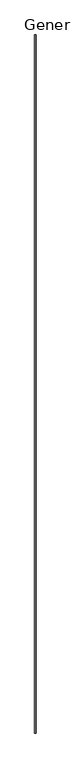
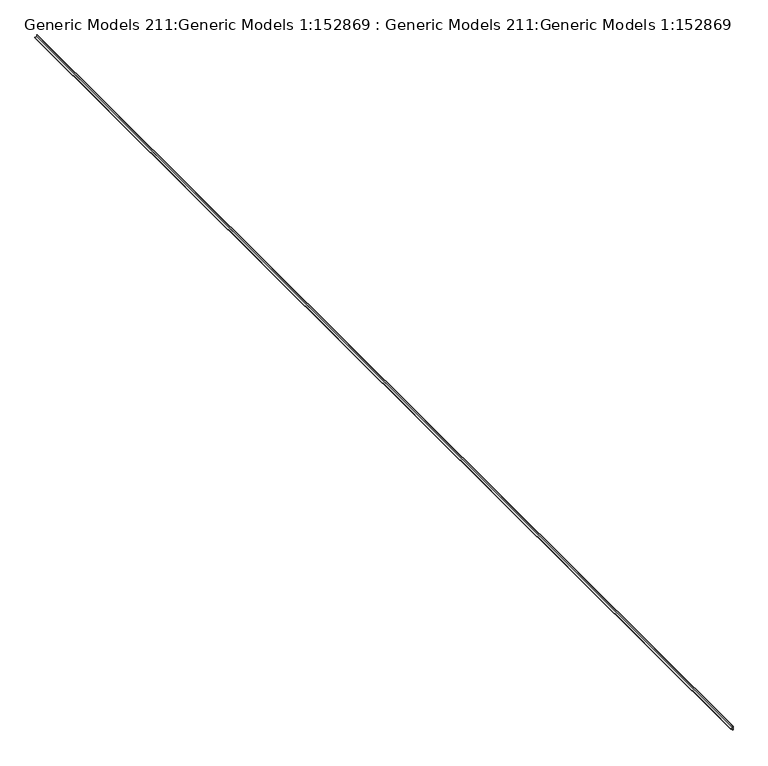
"""IFC4 building model written with IfcOpenShell, lengths in millimetres: proxy geometry, Generic Models 211:Generic Models 1:152869 : Generic Models 211:Generic Models 1:152869."""

from ifc_helpers import new_model, si_unit, frame, origin, place, context, project, spatial, polyline, outline, extrude, source, transform, mapped, element, save


def generic_models_211_generic_models_1_152869_generic_models_dbfa076a(model_context):
    return source(origin(), model_context, "Body", "SweptSolid", [
        extrude(outline(polyline([(3005.455, -6667.0793913), (3044.825, -6667.0793913), (3044.825, -6668.3493913), (3025.775, -6668.3493913), (3025.775, -6689.3043913), (3021.0252, -6689.3043913), (3021.0252, -6688.0343913), (3024.505, -6688.0343913), (3024.505, -6668.3493913), (3005.455, -6668.3493913), (3005.455, -6667.0793913)])), frame((0.0, -273.9974793, 0.0), z_axis=(0.0, 1.0, 0.0), x_axis=(0.0, 0.0, 1.0)), (0.0, 0.0, 1.0), 12446.0),
    ])


if __name__ == "__main__":
    model = new_model("IFC4")
    model_context = context("Model", 3, world=origin())
    ifc_project = project(units=[si_unit("LENGTHUNIT", "METRE", prefix="MILLI")], contexts=[model_context])
    site = spatial("IfcSite", under=ifc_project)
    building = spatial("IfcBuilding", under=site)
    placement = place(None, origin())
    generic_models_211_generic_models_1_152869_generic_models_shape = generic_models_211_generic_models_1_152869_generic_models_dbfa076a(model_context)
    element("IfcBuildingElementProxy", 1, Name="Generic Models 211:Generic Models 1:152869 : Generic Models 211:Generic Models 1:152869", ObjectType="Generic Models 211:Generic Models 1:152869 : Generic Models 211:Generic Models 1:152869", at=placement, inside=building, context=model_context, shape_type="MappedRepresentation", body=[
        mapped(generic_models_211_generic_models_1_152869_generic_models_shape, transform((0.0, 0.0, 0.0), x_axis=(1.0, 0.0, 0.0), y_axis=(0.0, 1.0, 0.0), z_axis=(0.0, 0.0, 1.0))),
    ])
    save(model, "model.ifc")

# Revit data of these elements
# Type "Generic Models 211:Generic Models 1:152869 : Generic Models 211:Generic Models 1:152869"
#   NameOverride = "Generic Models 211:Generic Models 1:152869"
#   ObjectTypeOverride = "Generic Models 211:Generic Models 1"
#   Reference = "Generic Models 1"
#   Category = "Generic Models"
#   Tag = "152869"
# Element 1 (IfcBuildingElementProxy, "Generic Models 211:Generic Models 1:152869 : Generic Models 211:Generic Models 1:152869")
#   Materials on its faces: "_ 16 GA. COPPER VENTED T REVEAL BEAD (CONT. AROUND PERIMETER OF BEAM) 2987"
# Materials
#   "_ 16 GA. COPPER VENTED T REVEAL BEAD (CONT. AROUND PERIMETER OF BEAM) 2987": class "Unassigned", colour RGB 253 192 103, transparency 0
